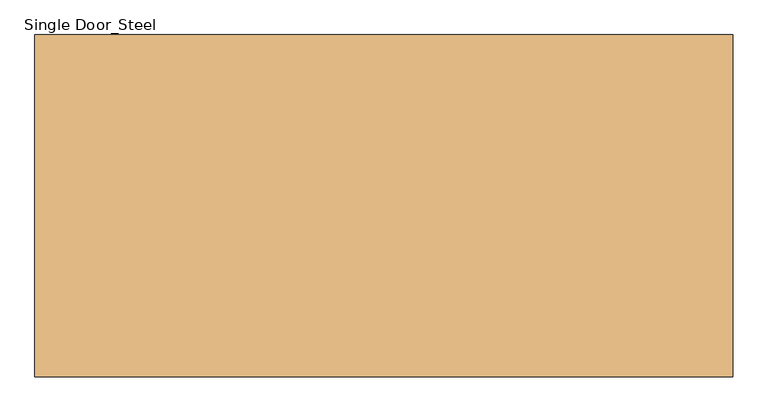
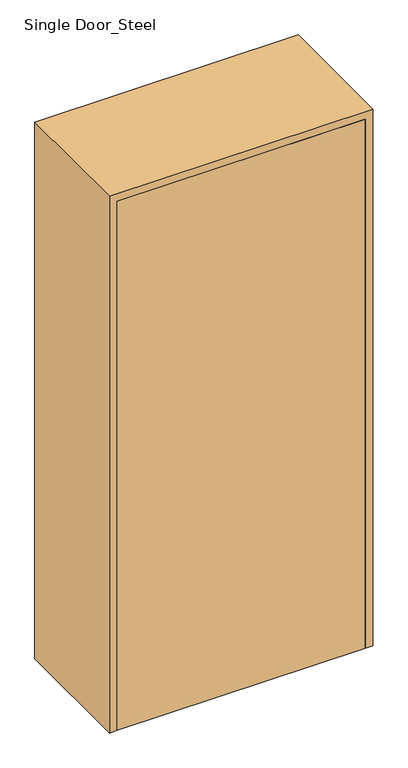
"""IFC4 building model written with IfcOpenShell, lengths in millimetres: door geometry, Single Door_Steel : H_DR_AMB_Single Door_Steel_W1000xH2150."""

import ifcopenshell
import ifcopenshell.guid

model = None  # the IFC model being written
_history = None  # IfcOwnerHistory: only IFC2X3 demands one
_inside = {}  # id of a spatial element -> (the spatial element, [elements in it])
_under = {}  # id of a project, library or spatial element -> (it, [spatial elements below it])
_declared = {}  # id of a project -> (the project, [libraries it declares])
_typed = {}  # id of a type object -> (the type object, [elements of that type])
_made_of = {}  # id of a material, layer set ... -> (it, [elements and type objects made of it])


def new_model(schema):
    """Start an empty IFC model of exactly this schema.

    Asked for "IFC4X3", IfcOpenShell would pick the latest addendum, in which some entities
    have other attributes; the version numbers below select the first issue.
    IFC2X3 requires an IfcOwnerHistory on every rooted entity: one is made here for all.
    """
    global model, _history
    if schema == "IFC4X3":
        model = ifcopenshell.file(schema_version=(4, 3, 0, 0))
    else:
        model = ifcopenshell.file(schema=schema)
    _inside.clear()
    _under.clear()
    _declared.clear()
    _typed.clear()
    _made_of.clear()
    _history = None
    if model.schema == "IFC2X3":
        org = make("IfcOrganization", Name="unknown")
        user = make(
            "IfcPersonAndOrganization",
            ThePerson=make("IfcPerson", FamilyName="unknown"),
            TheOrganization=org,
        )
        app = make(
            "IfcApplication",
            ApplicationDeveloper=org,
            Version="unknown",
            ApplicationFullName="unknown",
            ApplicationIdentifier="unknown",
        )
        _history = make(
            "IfcOwnerHistory",
            OwningUser=user,
            OwningApplication=app,
            ChangeAction="ADDED",
            CreationDate=0,
        )
    return model


def make(cls, **values):
    """One entity of the class cls with the attributes given. An attribute that is None is left unset."""
    return model.create_entity(
        cls, **{name: value for name, value in values.items() if value is not None}
    )


def rooted(cls, **values):
    """An entity with a GlobalId (a new one), such as an element, a storey or a relation."""
    return make(cls, GlobalId=ifcopenshell.guid.new(), OwnerHistory=_history, **values)


def si_unit(unit_type, name, prefix=None):
    """IfcSIUnit, for example si_unit("LENGTHUNIT", "METRE", prefix="MILLI")."""
    return make("IfcSIUnit", UnitType=unit_type, Prefix=prefix, Name=name)


def assignment(units):
    """IfcUnitAssignment: the units of a project."""
    return None if units is None else make("IfcUnitAssignment", Units=units)


def point(xyz):
    """IfcCartesianPoint."""
    return None if xyz is None else make("IfcCartesianPoint", Coordinates=xyz)


def direction(xyz):
    """IfcDirection."""
    return None if xyz is None else make("IfcDirection", DirectionRatios=xyz)


def frame(location, z_axis=None, x_axis=None):
    """IfcAxis2Placement3D, a coordinate frame: its origin and axes. An axis left out is left unset."""
    return make(
        "IfcAxis2Placement3D",
        Location=point(location),
        Axis=direction(z_axis),
        RefDirection=direction(x_axis),
    )


def origin():
    """The frame at (0, 0, 0) with its axes left unset."""
    return frame((0.0, 0.0, 0.0))


def origin_with_axes():
    """The frame at (0, 0, 0) with the z axis (0, 0, 1) and the x axis (1, 0, 0) written out."""
    return frame((0.0, 0.0, 0.0), z_axis=(0.0, 0.0, 1.0), x_axis=(1.0, 0.0, 0.0))


def place(relative_to, where):
    """IfcLocalPlacement: puts the frame where relative to a parent placement (None: the world)."""
    return make(
        "IfcLocalPlacement", PlacementRelTo=relative_to, RelativePlacement=where
    )


def context(
    kind, dimensions, precision=None, world=None, true_north=None, identifier=None
):
    """IfcGeometricRepresentationContext, for example the 3D "Model" context."""
    return make(
        "IfcGeometricRepresentationContext",
        ContextIdentifier=identifier,
        ContextType=kind,
        CoordinateSpaceDimension=dimensions,
        Precision=precision,
        WorldCoordinateSystem=world,
        TrueNorth=true_north,
    )


def project(units=None, contexts=None):
    """IfcProject with its units and contexts."""
    return rooted(
        "IfcProject",
        Name="project",
        RepresentationContexts=contexts,
        UnitsInContext=assignment(units),
    )


def spatial(cls, under=None, at=None, **own):
    """A site, building, storey or space (cls), placed at a placement, below another one or the project."""
    s = rooted(cls, ObjectPlacement=at, **own)
    if under is not None:
        _under.setdefault(under.id(), (under, []))[1].append(s)
    return s


def polyline(points):
    """IfcPolyline through the points."""
    return make("IfcPolyline", Points=[point(p) for p in points])


def outline(outer, holes=None, kind="AREA"):
    """IfcArbitraryClosedProfileDef: a profile drawn as a closed curve; with holes, ...WithVoids."""
    if holes is None:
        return make("IfcArbitraryClosedProfileDef", ProfileType=kind, OuterCurve=outer)
    return make(
        "IfcArbitraryProfileDefWithVoids",
        ProfileType=kind,
        OuterCurve=outer,
        InnerCurves=holes,
    )


def extrude(swept, where, along, depth):
    """IfcExtrudedAreaSolid: the profile swept, set in the frame where, extruded along a direction by depth."""
    return make(
        "IfcExtrudedAreaSolid",
        SweptArea=swept,
        Position=where,
        ExtrudedDirection=direction(along),
        Depth=depth,
    )


def faces_of(points, faces, orient=None, outer=None):
    """IfcFace entities. A face is a list of loops; a loop is a list of indices into points, from 0.

    orient and outer hold one flag for each loop. By default every Orientation is true, the
    first loop of a face is its IfcFaceOuterBound and the others are IfcFaceBound.
    """
    made = []
    for i, loops in enumerate(faces):
        bounds = []
        for j, loop in enumerate(loops):
            is_outer = j == 0 if outer is None else outer[i][j]
            bounds.append(
                make(
                    "IfcFaceOuterBound" if is_outer else "IfcFaceBound",
                    Bound=make("IfcPolyLoop", Polygon=[points[k] for k in loop]),
                    Orientation=True if orient is None else orient[i][j],
                )
            )
        made.append(make("IfcFace", Bounds=bounds))
    return made


def faceted_brep(points, faces, orient=None, outer=None, voids=None):
    """IfcFacetedBrep: a solid bounded by flat faces; with voids (closed shells), ...WithVoids."""
    shared = [point(p) for p in points]
    hull = make("IfcClosedShell", CfsFaces=faces_of(shared, faces, orient, outer))
    if voids is None:
        return make("IfcFacetedBrep", Outer=hull)
    return make(
        "IfcFacetedBrepWithVoids",
        Outer=hull,
        Voids=[
            make(cls, CfsFaces=faces_of(shared, fs, o, b)) for cls, fs, o, b in voids
        ],
    )


def shape(context_of_items, identifier, shape_type, items):
    """IfcShapeRepresentation: the items that make up one representation, for example the "Body"."""
    return make(
        "IfcShapeRepresentation",
        ContextOfItems=context_of_items,
        RepresentationIdentifier=identifier,
        RepresentationType=shape_type,
        Items=items,
    )


def source(mapping_origin, context_of_items, identifier, shape_type, items):
    """IfcRepresentationMap: a shape defined once, which mapped items show again and again."""
    return make(
        "IfcRepresentationMap",
        MappingOrigin=mapping_origin,
        MappedRepresentation=shape(context_of_items, identifier, shape_type, items),
    )


def transform(
    local_origin,
    x_axis=None,
    y_axis=None,
    z_axis=None,
    scale=None,
    scale2=None,
    scale3=None,
    uniform=True,
):
    """IfcCartesianTransformationOperator3D, or its non-uniform kind. x_axis, y_axis, z_axis: its Axis1, 2, 3."""
    if uniform:
        return make(
            "IfcCartesianTransformationOperator3D",
            Axis1=direction(x_axis),
            Axis2=direction(y_axis),
            LocalOrigin=point(local_origin),
            Scale=scale,
            Axis3=direction(z_axis),
        )
    return make(
        "IfcCartesianTransformationOperator3DnonUniform",
        Axis1=direction(x_axis),
        Axis2=direction(y_axis),
        LocalOrigin=point(local_origin),
        Scale=scale,
        Axis3=direction(z_axis),
        Scale2=scale2,
        Scale3=scale3,
    )


def mapped(mapping_source, mapping_target):
    """IfcMappedItem: shows the shape of a source again, moved by a transform."""
    return make(
        "IfcMappedItem", MappingSource=mapping_source, MappingTarget=mapping_target
    )


def made_of(thing, what):
    """Note that an element or type object is made of a material, layer set ...; save() writes the relation."""
    if what is not None:
        _made_of.setdefault(what.id(), (what, []))[1].append(thing)
    return thing


def element(
    cls,
    number,
    at=None,
    inside=None,
    cuts=None,
    type_object=None,
    material=None,
    context=None,
    identifier="Body",
    shape_type=None,
    held_by="IfcProductDefinitionShape",
    body=None,
    shapes=None,
    **own,
):
    """One element of the class cls, such as IfcWall. Its Tag is "e" and its number.

    at: its placement. inside: the storey or other place that contains it. cuts: it is an
    opening in that element (IfcRelVoidsElement). A single representation is given by context,
    identifier, shape_type and body (its items); several are given by shapes. held_by: the class
    of the entity that holds the representations. save() writes the other relations.
    """
    e = rooted(cls, Tag="e%d" % number, ObjectPlacement=at, **own)
    if body is not None:
        shapes = [shape(context, identifier, shape_type, body)]
    if shapes is not None:
        e.Representation = make(held_by, Representations=shapes)
    if inside is not None:
        _inside.setdefault(inside.id(), (inside, []))[1].append(e)
    if cuts is not None:
        rooted(
            "IfcRelVoidsElement", RelatingBuildingElement=cuts, RelatedOpeningElement=e
        )
    if type_object is not None:
        _typed.setdefault(type_object.id(), (type_object, []))[1].append(e)
    return made_of(e, material)


def aggregate(whole, parts):
    """IfcRelAggregates: a whole, such as a stair, and the parts it consists of."""
    return rooted("IfcRelAggregates", RelatingObject=whole, RelatedObjects=parts)


def save(model, path):
    """Write the relations noted so far, then the file.

    IfcRelAggregates (storeys below a building ...), IfcRelContainedInSpatialStructure (elements
    in a storey), IfcRelDefinesByType, IfcRelAssociatesMaterial and IfcRelDeclares: one each for
    every whole, place, type object, material and project.
    """
    for whole, parts in _under.values():
        aggregate(whole, parts)
    for where, things in _inside.values():
        rooted(
            "IfcRelContainedInSpatialStructure",
            RelatedElements=things,
            RelatingStructure=where,
        )
    for kind, things in _typed.values():
        rooted("IfcRelDefinesByType", RelatedObjects=things, RelatingType=kind)
    for what, things in _made_of.values():
        rooted("IfcRelAssociatesMaterial", RelatedObjects=things, RelatingMaterial=what)
    for by, libraries in _declared.values():
        rooted("IfcRelDeclares", RelatingContext=by, RelatedDefinitions=libraries)
    model.write(path)


def single_door_steel_cad2a4f8(model_context):
    return source(origin(), model_context, "Body", "SolidModel", [
        extrude(outline(polyline([(470.0, -245.0), (-470.0, -245.0), (-470.0, -210.0), (470.0, -210.0), (470.0, -245.0)])), origin_with_axes(), (0.0, 0.0, 1.0), 2120.0),
        faceted_brep([(470.0, -245.0, 0.0), (470.0, -210.0, 0.0), (450.0, -210.0, 0.0), (450.0, 210.0, 0.0), (470.0, 210.0, 0.0), (470.0, 245.0, 0.0), (500.0, 245.0, 0.0), (500.0, -245.0, 0.0), (500.0, -245.0, 2150.0), (-500.0, -245.0, 2150.0), (-500.0, -245.0, 0.0), (-470.0, -245.0, 0.0), (-470.0, -245.0, 2120.0), (470.0, -245.0, 2120.0), (500.0, 245.0, 2150.0), (470.0, 245.0, 2120.0), (-470.0, 245.0, 2120.0), (-470.0, 245.0, 0.0), (-500.0, 245.0, 0.0), (-500.0, 245.0, 2150.0), (470.0, 210.0, 2120.0), (450.0, 210.0, 2100.0), (-450.0, 210.0, 2100.0), (-450.0, 210.0, 0.0), (-470.0, 210.0, 0.0), (-470.0, 210.0, 2120.0), (450.0, -210.0, 2100.0), (470.0, -210.0, 2120.0), (-470.0, -210.0, 2120.0), (-470.0, -210.0, 0.0), (-450.0, -210.0, 0.0), (-450.0, -210.0, 2100.0)], [[[0, 1, 2, 3, 4, 5, 6, 7]], [[7, 8, 9, 10, 11, 12, 13, 0]], [[6, 14, 8, 7]], [[5, 15, 16, 17, 18, 19, 14, 6]], [[4, 20, 15, 5]], [[3, 21, 22, 23, 24, 25, 20, 4]], [[2, 26, 21, 3]], [[1, 27, 28, 29, 30, 31, 26, 2]], [[0, 13, 27, 1]], [[12, 11, 29, 28]], [[11, 10, 18, 17, 24, 23, 30, 29]], [[19, 18, 10, 9]], [[25, 24, 17, 16]], [[31, 30, 23, 22]], [[14, 19, 9, 8]], [[20, 25, 16, 15]], [[26, 31, 22, 21]], [[13, 12, 28, 27]]]),
    ])


if __name__ == "__main__":
    model = new_model("IFC4")
    model_context = context("Model", 3, world=origin())
    ifc_project = project(units=[si_unit("LENGTHUNIT", "METRE", prefix="MILLI")], contexts=[model_context])
    site = spatial("IfcSite", under=ifc_project)
    building = spatial("IfcBuilding", under=site)
    placement = place(None, origin())
    single_door_steel_shape = single_door_steel_cad2a4f8(model_context)
    element("IfcDoor", 1, ObjectType="Single Door_Steel : H_DR_AMB_Single Door_Steel_W1000xH2150", at=placement, inside=building, context=model_context, shape_type="MappedRepresentation", body=[
        mapped(single_door_steel_shape, transform((0.0, 0.0, 0.0), x_axis=(1.0, 0.0, 0.0), y_axis=(0.0, 1.0, 0.0), z_axis=(0.0, 0.0, 1.0))),
    ])
    save(model, "model.ifc")

# Revit data of these elements
# Type "Single Door_Steel : H_DR_AMB_Single Door_Steel_W1000xH2150"
#   Type Mark = "364"
#   Analytic Construction = "<None>"
#   프레임 투영 외부. = 25.000 mm
#   프레임 투영 내부. = 25.000 mm
#   프레임 폭 = 75.000 mm
#   Height = 2150.000 mm
#   Width = 1000.000 mm
#   Define Thermal Properties by = 1
#   문 패널 = none
#   문 프레임 = none
#   Function = (empty or 0)
#   Wall Closure = (empty or 0)
